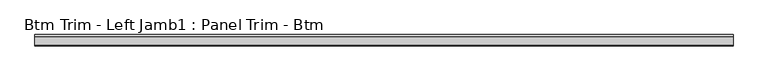
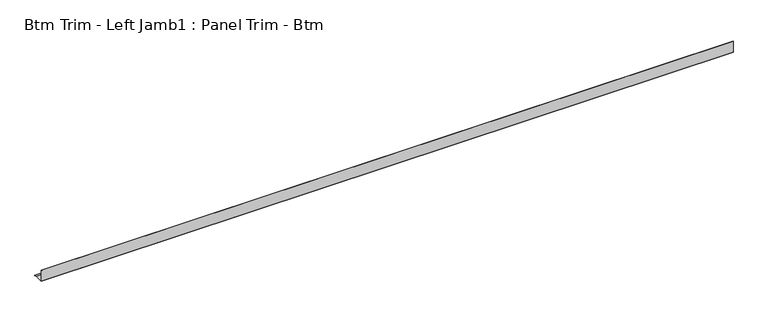
"""IFC4 building model written with IfcOpenShell, lengths in millimetres: proxy geometry, Btm Trim - Left Jamb1 : Panel Trim - Btm."""

from ifc_helpers import new_model, si_unit, frame, origin, place, context, project, spatial, polyline, outline, extrude, source, transform, mapped, element, save


def btm_trim_left_jamb1_panel_trim_btm_b9c60ca2(model_context):
    return source(origin(), model_context, "Body", "SweptSolid", [
        extrude(outline(polyline([(-531600.2244849, 0.79375), (-531590.923103, -1.6985478), (-531591.1285406, -2.4652514), (-531600.3289841, 0.0), (-531640.0037841, 0.0), (-531640.0037841, 51.59375), (-531639.2163841, 51.59375), (-531639.2163841, 0.79375), (-531600.2244849, 0.79375)])), frame((587327.7998239, 0.0, 0.0), z_axis=(1.0, 0.0, 0.0), x_axis=(0.0, 1.0, 0.0)), (0.0, 0.0, 1.0), 3063.2733375),
    ])


if __name__ == "__main__":
    model = new_model("IFC4")
    model_context = context("Model", 3, world=origin())
    ifc_project = project(units=[si_unit("LENGTHUNIT", "METRE", prefix="MILLI")], contexts=[model_context])
    site = spatial("IfcSite", under=ifc_project)
    building = spatial("IfcBuilding", under=site)
    placement = place(None, origin())
    btm_trim_left_jamb1_panel_trim_btm_shape = btm_trim_left_jamb1_panel_trim_btm_b9c60ca2(model_context)
    element("IfcBuildingElementProxy", 1, Name="Btm Trim - Left Jamb1 : Panel Trim - Btm", ObjectType="Btm Trim - Left Jamb1 : Panel Trim - Btm", at=placement, inside=building, context=model_context, shape_type="MappedRepresentation", body=[
        mapped(btm_trim_left_jamb1_panel_trim_btm_shape, transform((0.0, 0.0, 0.0), x_axis=(1.0, 0.0, 0.0), y_axis=(0.0, 1.0, 0.0), z_axis=(0.0, 0.0, 1.0))),
    ])
    save(model, "model.ifc")

# Revit data of these elements
# Element 1 (IfcBuildingElementProxy, "Btm Trim - Left Jamb1 : Panel Trim - Btm")
#   Materials on its faces: "BASE TRIM BY MTL PANEL MFR."
# Materials
#   "BASE TRIM BY MTL PANEL MFR.": class "Generic", colour RGB 239 242 240, transparency 0, Cost = 0
